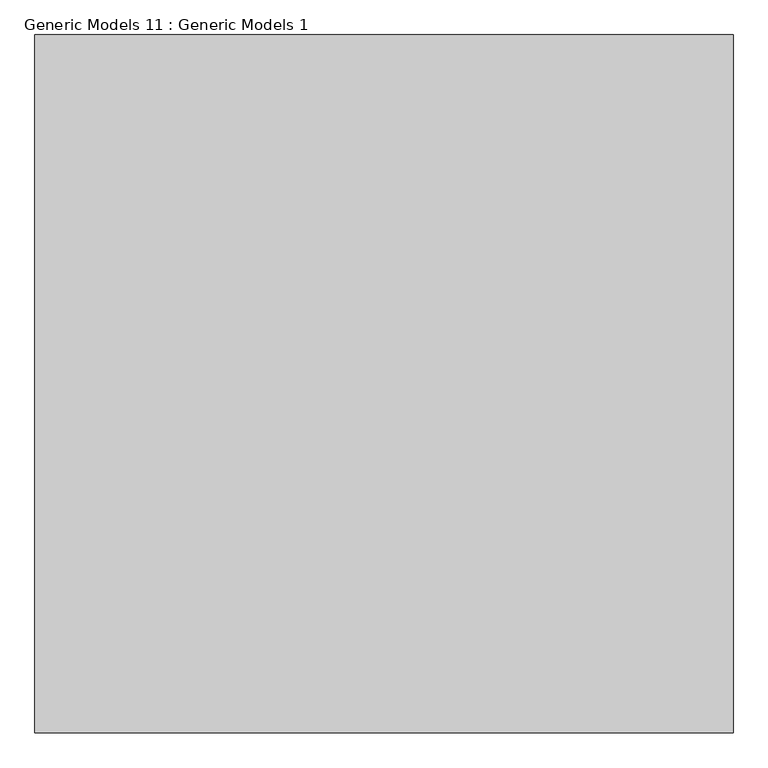
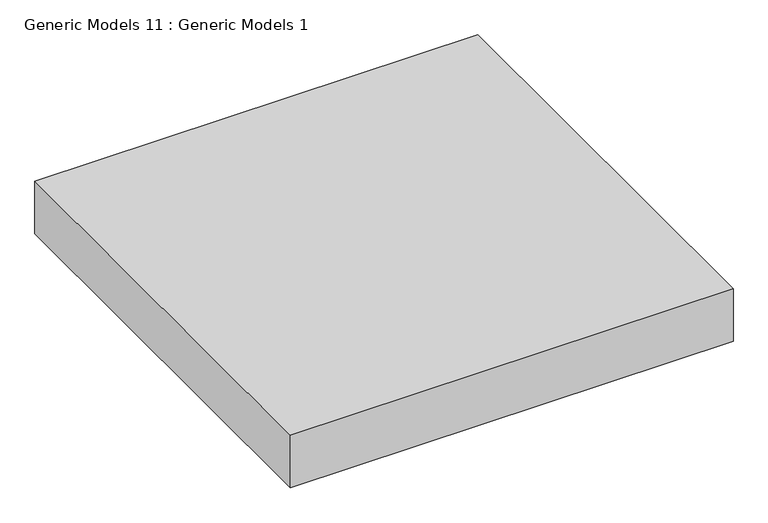
"""IFC4 building model written with IfcOpenShell, lengths in millimetres: proxy geometry, Generic Models 11 : Generic Models 1."""

from ifc_helpers import new_model, si_unit, frame, origin, place, context, project, spatial, polyline, outline, extrude, source, transform, mapped, element, save


def generic_models_11_generic_models_1_850b304e(model_context):
    return source(origin(), model_context, "Body", "SweptSolid", [
        extrude(outline(polyline([(50347.5625, 0.0), (49128.3625, 0.0), (49128.3625, 1219.2), (50347.5625, 1219.2), (50347.5625, 0.0)])), frame((0.0, 0.0, -152.4), z_axis=(0.0, 0.0, 1.0), x_axis=(1.0, 0.0, 0.0)), (0.0, 0.0, 1.0), 152.4),
    ])


if __name__ == "__main__":
    model = new_model("IFC4")
    model_context = context("Model", 3, world=origin())
    ifc_project = project(units=[si_unit("LENGTHUNIT", "METRE", prefix="MILLI")], contexts=[model_context])
    site = spatial("IfcSite", under=ifc_project)
    building = spatial("IfcBuilding", under=site)
    placement = place(None, origin())
    generic_models_11_generic_models_1_shape = generic_models_11_generic_models_1_850b304e(model_context)
    element("IfcBuildingElementProxy", 1, Name="Generic Models 11 : Generic Models 1", ObjectType="Generic Models 11 : Generic Models 1", at=placement, inside=building, context=model_context, shape_type="MappedRepresentation", body=[
        mapped(generic_models_11_generic_models_1_shape, transform((0.0, 0.0, 0.0), x_axis=(1.0, 0.0, 0.0), y_axis=(0.0, 1.0, 0.0), z_axis=(0.0, 0.0, 1.0))),
    ])
    save(model, "model.ifc")

# Revit data of these elements
# Element 1 (IfcBuildingElementProxy, "Generic Models 11 : Generic Models 1")
#   Materials on its faces: "STRUCTURAL FLOOR"
# Materials
#   "STRUCTURAL FLOOR": class "Concrete", colour RGB 36 37 33, transparency 0, Description = "Lightweight concrete", Cost = 0
